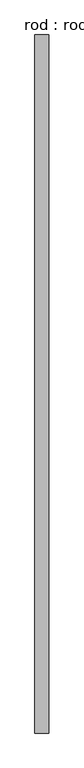
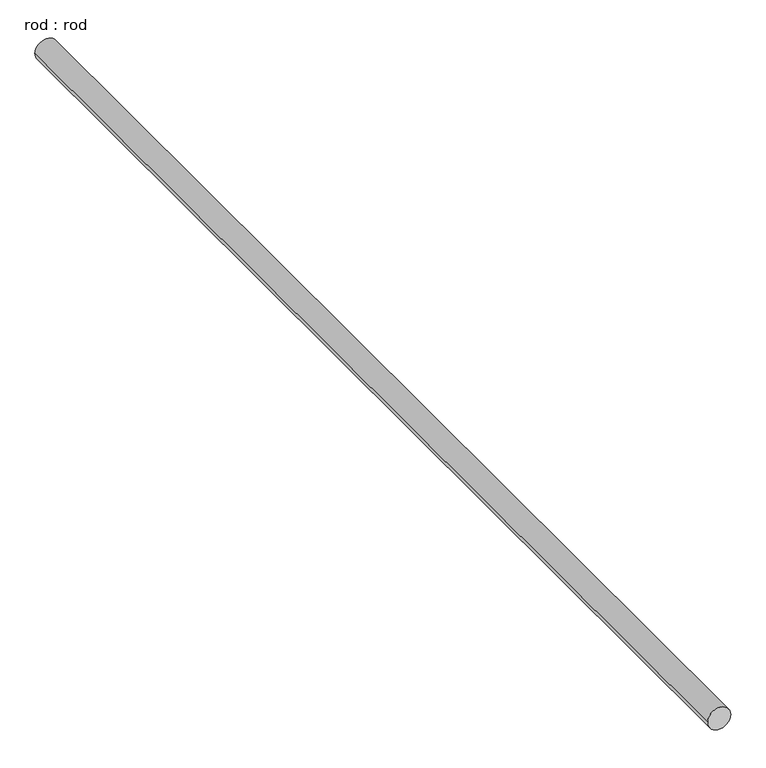
"""IFC4 building model written with IfcOpenShell, lengths in millimetres: proxy geometry, rod : rod."""

from ifc_helpers import new_model, si_unit, point, frame, frame_2d, origin, place, context, project, spatial, circle_curve, trimmed, segment, composite_curve, outline, extrude, source, transform, mapped, element, save


def rod_rod_2f70e640(model_context):
    return source(origin(), model_context, "Body", "SweptSolid", [
        extrude(outline(composite_curve([segment(trimmed(circle_curve(frame_2d((0.0108462, 0.0)), 200.0), [point((0.0108462, 200.0))], [point((0.0108462, -200.0))], False, "CARTESIAN"), True, "CONTINUOUS"), segment(trimmed(circle_curve(frame_2d((0.0108462, 0.0)), 200.0), [point((0.0108462, -200.0))], [point((0.0108462, 200.0))], False, "CARTESIAN"), True, "CONTINUOUS")], self_intersect=False)), frame((0.0, -6032.2713847, 0.0), z_axis=(0.0, 1.0, 0.0), x_axis=(0.0, 0.0, 1.0)), (0.0, 0.0, 1.0), 20250.0),
    ])


if __name__ == "__main__":
    model = new_model("IFC4")
    model_context = context("Model", 3, world=origin())
    ifc_project = project(units=[si_unit("LENGTHUNIT", "METRE", prefix="MILLI")], contexts=[model_context])
    site = spatial("IfcSite", under=ifc_project)
    building = spatial("IfcBuilding", under=site)
    placement = place(None, origin())
    rod_rod_shape = rod_rod_2f70e640(model_context)
    element("IfcBuildingElementProxy", 1, Name="rod : rod", ObjectType="rod : rod", at=placement, inside=building, context=model_context, shape_type="MappedRepresentation", body=[
        mapped(rod_rod_shape, transform((0.0, 0.0, 0.0), x_axis=(1.0, 0.0, 0.0), y_axis=(0.0, 1.0, 0.0), z_axis=(0.0, 0.0, 1.0))),
    ])
    save(model, "model.ifc")

# Revit data of these elements
# Type "rod : rod"
#   Default Elevation = 0
